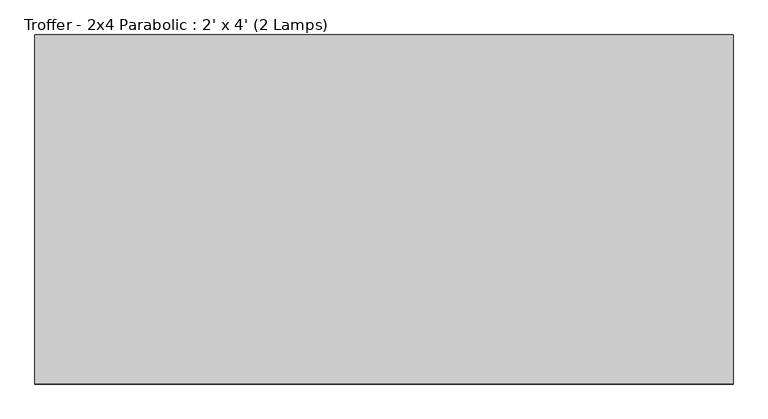
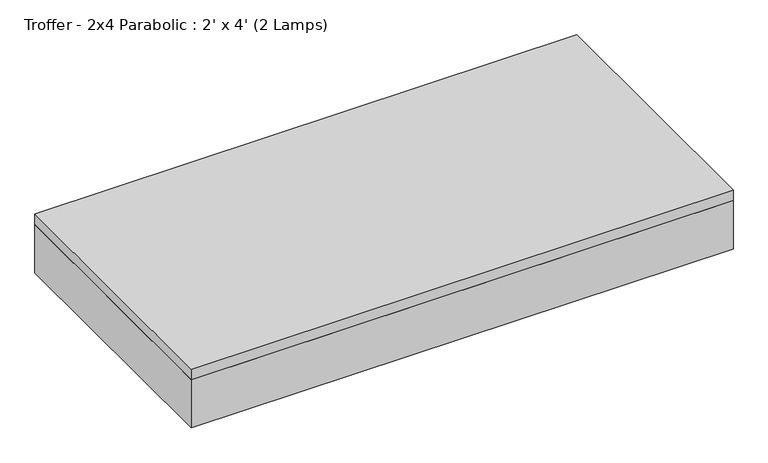
"""IFC4 building model written with IfcOpenShell, lengths in millimetres: light fixture geometry, Troffer - 2x4 Parabolic : 2' x 4' (2 Lamps)."""

from ifc_helpers import new_model, si_unit, frame, origin, place, context, project, spatial, polyline, outline, extrude, source, transform, mapped, element, save


def troffer_2x4_parabolic_2_x_4_2_lamps_ca384779(model_context):
    return source(origin(), model_context, "Body", "SweptSolid", [
        extrude(outline(polyline([(565.4964984, 219.9340679), (565.4964984, -338.8659321), (-602.9035016, -338.8659321), (-602.9035016, 219.9340679), (565.4964984, 219.9340679)]), holes=[polyline([(-409.2285016, 35.7840679), (-409.2285016, 213.5840679), (-596.5535016, 213.5840679), (-596.5535016, 35.7840679), (-409.2285016, 35.7840679)]), polyline([(-409.2285016, -148.3659321), (-409.2285016, 29.4340679), (-596.5535016, 29.4340679), (-596.5535016, -148.3659321), (-409.2285016, -148.3659321)]), polyline([(-409.2285016, -154.7159321), (-596.5535016, -154.7159321), (-596.5535016, -332.5159321), (-409.2285016, -332.5159321), (-409.2285016, -154.7159321)]), polyline([(-215.5535016, 35.7840679), (-215.5535016, 213.5840679), (-402.8785016, 213.5840679), (-402.8785016, 35.7840679), (-215.5535016, 35.7840679)]), polyline([(-215.5535016, -148.3659321), (-215.5535016, 29.4340679), (-402.8785016, 29.4340679), (-402.8785016, -148.3659321), (-215.5535016, -148.3659321)]), polyline([(-215.5535016, -154.7159321), (-402.8785016, -154.7159321), (-402.8785016, -332.5159321), (-215.5535016, -332.5159321), (-215.5535016, -154.7159321)]), polyline([(-21.8785016, 35.7840679), (-21.8785016, 213.5840679), (-209.2035016, 213.5840679), (-209.2035016, 35.7840679), (-21.8785016, 35.7840679)]), polyline([(-21.8785016, -148.3659321), (-21.8785016, 29.4340679), (-209.2035016, 29.4340679), (-209.2035016, -148.3659321), (-21.8785016, -148.3659321)]), polyline([(-21.8785016, -154.7159321), (-209.2035016, -154.7159321), (-209.2035016, -332.5159321), (-21.8785016, -332.5159321), (-21.8785016, -154.7159321)]), polyline([(171.7964984, 35.7840679), (171.7964984, 213.5840679), (-15.5285016, 213.5840679), (-15.5285016, 35.7840679), (171.7964984, 35.7840679)]), polyline([(171.7964984, -148.3659321), (171.7964984, 29.4340679), (-15.5285016, 29.4340679), (-15.5285016, -148.3659321), (171.7964984, -148.3659321)]), polyline([(171.7964984, -154.7159321), (-15.5285016, -154.7159321), (-15.5285016, -332.5159321), (171.7964984, -332.5159321), (171.7964984, -154.7159321)]), polyline([(365.4714984, 35.7840679), (365.4714984, 213.5840679), (178.1464984, 213.5840679), (178.1464984, 35.7840679), (365.4714984, 35.7840679)]), polyline([(365.4714984, -148.3659321), (365.4714984, 29.4340679), (178.1464984, 29.4340679), (178.1464984, -148.3659321), (365.4714984, -148.3659321)]), polyline([(365.4714984, -154.7159321), (178.1464984, -154.7159321), (178.1464984, -332.5159321), (365.4714984, -332.5159321), (365.4714984, -154.7159321)]), polyline([(559.1464984, 35.7840679), (559.1464984, 213.5840679), (371.8214984, 213.5840679), (371.8214984, 35.7840679), (559.1464984, 35.7840679)]), polyline([(559.1464984, -148.3659321), (559.1464984, 29.4340679), (371.8214984, 29.4340679), (371.8214984, -148.3659321), (559.1464984, -148.3659321)]), polyline([(559.1464984, -154.7159321), (371.8214984, -154.7159321), (371.8214984, -332.5159321), (559.1464984, -332.5159321), (559.1464984, -154.7159321)])]), frame((0.0, 0.0, 2438.4), z_axis=(0.0, 0.0, 1.0), x_axis=(1.0, 0.0, 0.0)), (0.0, 0.0, 1.0), 3.175),
        extrude(outline(polyline([(565.4964984, 219.9340679), (565.4964984, -338.8659321), (-602.9035016, -338.8659321), (-602.9035016, 219.9340679), (565.4964984, 219.9340679)])), frame((0.0, 0.0, 2514.6), z_axis=(0.0, 0.0, 1.0), x_axis=(1.0, 0.0, 0.0)), (0.0, 0.0, 1.0), 6.35),
        extrude(outline(polyline([(565.4964984, 219.9340679), (565.4964984, -338.8659321), (-602.9035016, -338.8659321), (-602.9035016, 219.9340679), (565.4964984, 219.9340679)]), holes=[polyline([(-409.2285016, 35.7840679), (-409.2285016, 213.5840679), (-596.5535016, 213.5840679), (-596.5535016, 35.7840679), (-409.2285016, 35.7840679)]), polyline([(-409.2285016, -148.3659321), (-409.2285016, 29.4340679), (-596.5535016, 29.4340679), (-596.5535016, -148.3659321), (-409.2285016, -148.3659321)]), polyline([(-409.2285016, -154.7159321), (-596.5535016, -154.7159321), (-596.5535016, -332.5159321), (-409.2285016, -332.5159321), (-409.2285016, -154.7159321)]), polyline([(-215.5535016, 35.7840679), (-215.5535016, 213.5840679), (-402.8785016, 213.5840679), (-402.8785016, 35.7840679), (-215.5535016, 35.7840679)]), polyline([(-215.5535016, -148.3659321), (-215.5535016, 29.4340679), (-402.8785016, 29.4340679), (-402.8785016, -148.3659321), (-215.5535016, -148.3659321)]), polyline([(-215.5535016, -154.7159321), (-402.8785016, -154.7159321), (-402.8785016, -332.5159321), (-215.5535016, -332.5159321), (-215.5535016, -154.7159321)]), polyline([(-21.8785016, 35.7840679), (-21.8785016, 213.5840679), (-209.2035016, 213.5840679), (-209.2035016, 35.7840679), (-21.8785016, 35.7840679)]), polyline([(-21.8785016, -148.3659321), (-21.8785016, 29.4340679), (-209.2035016, 29.4340679), (-209.2035016, -148.3659321), (-21.8785016, -148.3659321)]), polyline([(-21.8785016, -154.7159321), (-209.2035016, -154.7159321), (-209.2035016, -332.5159321), (-21.8785016, -332.5159321), (-21.8785016, -154.7159321)]), polyline([(171.7964984, 35.7840679), (171.7964984, 213.5840679), (-15.5285016, 213.5840679), (-15.5285016, 35.7840679), (171.7964984, 35.7840679)]), polyline([(171.7964984, -148.3659321), (171.7964984, 29.4340679), (-15.5285016, 29.4340679), (-15.5285016, -148.3659321), (171.7964984, -148.3659321)]), polyline([(171.7964984, -154.7159321), (-15.5285016, -154.7159321), (-15.5285016, -332.5159321), (171.7964984, -332.5159321), (171.7964984, -154.7159321)]), polyline([(365.4714984, 35.7840679), (365.4714984, 213.5840679), (178.1464984, 213.5840679), (178.1464984, 35.7840679), (365.4714984, 35.7840679)]), polyline([(365.4714984, -148.3659321), (365.4714984, 29.4340679), (178.1464984, 29.4340679), (178.1464984, -148.3659321), (365.4714984, -148.3659321)]), polyline([(365.4714984, -154.7159321), (178.1464984, -154.7159321), (178.1464984, -332.5159321), (365.4714984, -332.5159321), (365.4714984, -154.7159321)]), polyline([(559.1464984, 35.7840679), (559.1464984, 213.5840679), (371.8214984, 213.5840679), (371.8214984, 35.7840679), (559.1464984, 35.7840679)]), polyline([(559.1464984, -148.3659321), (559.1464984, 29.4340679), (371.8214984, 29.4340679), (371.8214984, -148.3659321), (559.1464984, -148.3659321)]), polyline([(559.1464984, -154.7159321), (371.8214984, -154.7159321), (371.8214984, -332.5159321), (559.1464984, -332.5159321), (559.1464984, -154.7159321)])]), frame((0.0, 0.0, 2441.575), z_axis=(0.0, 0.0, 1.0), x_axis=(1.0, 0.0, 0.0)), (0.0, 0.0, 1.0), 47.625),
        extrude(outline(polyline([(590.8964984, 245.3340679), (590.8964984, -364.2659321), (-628.3035016, -364.2659321), (-628.3035016, 245.3340679), (590.8964984, 245.3340679)]), holes=[polyline([(565.4964984, 219.9340679), (-602.9035016, 219.9340679), (-602.9035016, -338.8659321), (565.4964984, -338.8659321), (565.4964984, 219.9340679)])]), frame((0.0, 0.0, 2438.4), z_axis=(0.0, 0.0, 1.0), x_axis=(1.0, 0.0, 0.0)), (0.0, 0.0, 1.0), 114.3),
        extrude(outline(polyline([(590.8964984, 245.3340679), (590.8964984, -364.2659321), (-628.3035016, -364.2659321), (-628.3035016, 245.3340679), (590.8964984, 245.3340679)])), frame((0.0, 0.0, 2552.7), z_axis=(0.0, 0.0, 1.0), x_axis=(1.0, 0.0, 0.0)), (0.0, 0.0, 1.0), 25.4),
    ])


if __name__ == "__main__":
    model = new_model("IFC4")
    model_context = context("Model", 3, world=origin())
    ifc_project = project(units=[si_unit("LENGTHUNIT", "METRE", prefix="MILLI")], contexts=[model_context])
    site = spatial("IfcSite", under=ifc_project)
    building = spatial("IfcBuilding", under=site)
    placement = place(None, origin())
    troffer_2x4_parabolic_2_x_4_2_lamps_shape = troffer_2x4_parabolic_2_x_4_2_lamps_ca384779(model_context)
    element("IfcLightFixture", 1, ObjectType="Troffer - 2x4 Parabolic : 2' x 4' (2 Lamps)", at=placement, inside=building, context=model_context, shape_type="MappedRepresentation", body=[
        mapped(troffer_2x4_parabolic_2_x_4_2_lamps_shape, transform((0.0, 0.0, 0.0), x_axis=(1.0, 0.0, 0.0), y_axis=(0.0, 1.0, 0.0), z_axis=(0.0, 0.0, 1.0))),
    ])
    save(model, "model.ifc")

# Revit data of these elements
# Type "Troffer - 2x4 Parabolic : 2' x 4' (2 Lamps)"
#   Assembly Code = "D5020210"
#   Lamp = "T-12"
#   Wattage Comments = "(2)20"
#   Wattage = 16.1571 W
#   built-in parameter 1150110 = 1 (stored number, unit not read)
#   built-in parameter 1114217 = 1 (stored number, unit not read)
#   built-in parameter 1150109 = 1 (stored number, unit not read)
#   built-in parameter 1150113 = 1 (stored number, unit not read)
#   built-in parameter 1150105 = 190.986 (stored number, unit not read)
#   built-in parameter 1150115 = 1 (stored number, unit not read)
#   Light Source Symbol Size = 2' - 0"
#   built-in parameter 1150112 = 1 (stored number, unit not read)
#   built-in parameter 1150114 = 1 (stored number, unit not read)
#   built-in parameter 1150107 = 3200 (stored number, unit not read)
#   built-in parameter 1150106 = 1.90986 (stored number, unit not read)
#   Emit from Line Length = 3' - 10"
#   built-in parameter 1150104 = 13.8 (stored number, unit not read)
#   built-in parameter 1114218 = 1 (stored number, unit not read)
#   built-in parameter 1150133 = 10 (stored number, unit not read)
#   Circle Width = 1' - 2.4"
#   Length = 4' - 0"
#   Lumens = 2400 lm
#   Width = 2' - 0"
#   built-in parameter 1150134 = 3
#   built-in parameter 1150132 = 2
#   Color Filter = 16777215
#   Diffuser = none
#   Light Box = none
#   Dimming Lamp Color Temperature Shift = (empty or 0)
